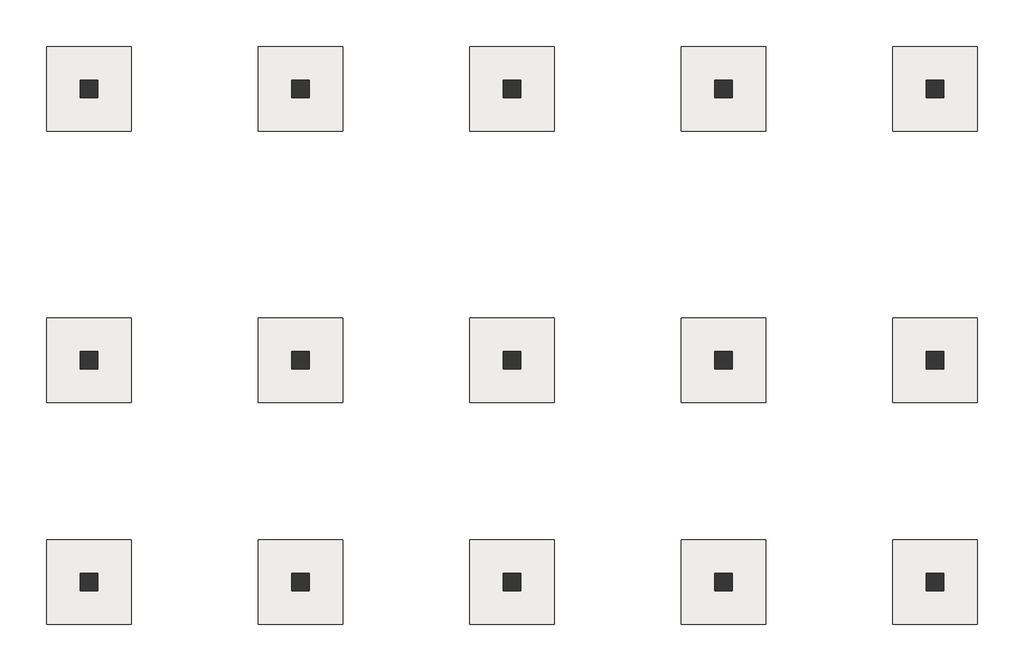
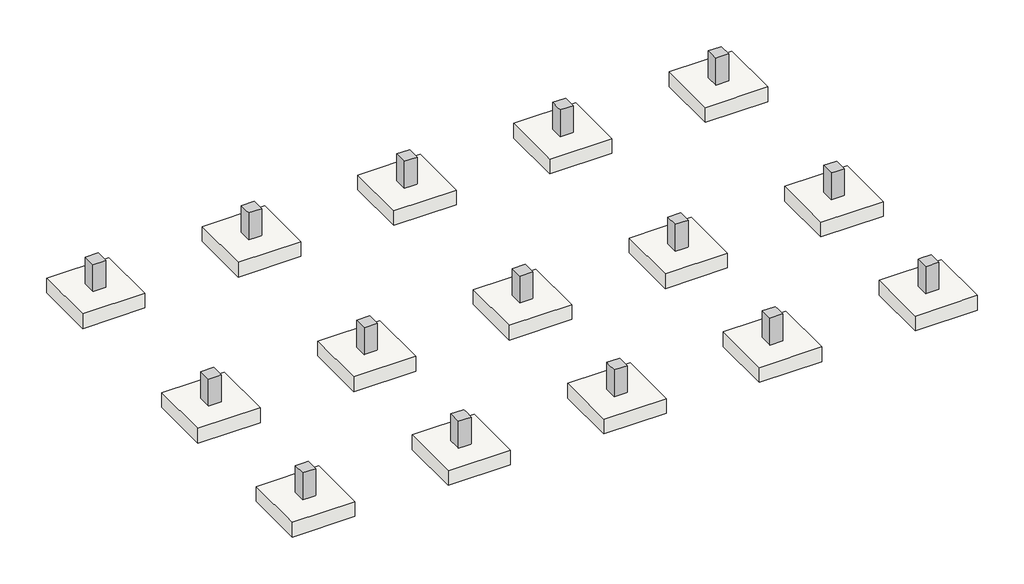
# One storey: 15 columns, 15 slabs.
"""IFC4 building model written with IfcOpenShell, lengths in millimetres."""

import ifcopenshell
import ifcopenshell.guid

model = None  # the IFC model being written
_history = None  # IfcOwnerHistory: only IFC2X3 demands one
_inside = {}  # id of a spatial element -> (the spatial element, [elements in it])
_under = {}  # id of a project, library or spatial element -> (it, [spatial elements below it])
_declared = {}  # id of a project -> (the project, [libraries it declares])
_typed = {}  # id of a type object -> (the type object, [elements of that type])
_made_of = {}  # id of a material, layer set ... -> (it, [elements and type objects made of it])


def new_model(schema):
    """Start an empty IFC model of exactly this schema.

    Asked for "IFC4X3", IfcOpenShell would pick the latest addendum, in which some entities
    have other attributes; the version numbers below select the first issue.
    IFC2X3 requires an IfcOwnerHistory on every rooted entity: one is made here for all.
    """
    global model, _history
    if schema == "IFC4X3":
        model = ifcopenshell.file(schema_version=(4, 3, 0, 0))
    else:
        model = ifcopenshell.file(schema=schema)
    _inside.clear()
    _under.clear()
    _declared.clear()
    _typed.clear()
    _made_of.clear()
    _history = None
    if model.schema == "IFC2X3":
        org = make("IfcOrganization", Name="unknown")
        user = make(
            "IfcPersonAndOrganization",
            ThePerson=make("IfcPerson", FamilyName="unknown"),
            TheOrganization=org,
        )
        app = make(
            "IfcApplication",
            ApplicationDeveloper=org,
            Version="unknown",
            ApplicationFullName="unknown",
            ApplicationIdentifier="unknown",
        )
        _history = make(
            "IfcOwnerHistory",
            OwningUser=user,
            OwningApplication=app,
            ChangeAction="ADDED",
            CreationDate=0,
        )
    return model


def make(cls, **values):
    """One entity of the class cls with the attributes given. An attribute that is None is left unset."""
    return model.create_entity(
        cls, **{name: value for name, value in values.items() if value is not None}
    )


def rooted(cls, **values):
    """An entity with a GlobalId (a new one), such as an element, a storey or a relation."""
    return make(cls, GlobalId=ifcopenshell.guid.new(), OwnerHistory=_history, **values)


def si_unit(unit_type, name, prefix=None):
    """IfcSIUnit, for example si_unit("LENGTHUNIT", "METRE", prefix="MILLI")."""
    return make("IfcSIUnit", UnitType=unit_type, Prefix=prefix, Name=name)


def assignment(units):
    """IfcUnitAssignment: the units of a project."""
    return None if units is None else make("IfcUnitAssignment", Units=units)


def point(xyz):
    """IfcCartesianPoint."""
    return None if xyz is None else make("IfcCartesianPoint", Coordinates=xyz)


def direction(xyz):
    """IfcDirection."""
    return None if xyz is None else make("IfcDirection", DirectionRatios=xyz)


def frame(location, z_axis=None, x_axis=None):
    """IfcAxis2Placement3D, a coordinate frame: its origin and axes. An axis left out is left unset."""
    return make(
        "IfcAxis2Placement3D",
        Location=point(location),
        Axis=direction(z_axis),
        RefDirection=direction(x_axis),
    )


def origin():
    """The frame at (0, 0, 0) with its axes left unset."""
    return frame((0.0, 0.0, 0.0))


def place(relative_to, where):
    """IfcLocalPlacement: puts the frame where relative to a parent placement (None: the world)."""
    return make(
        "IfcLocalPlacement", PlacementRelTo=relative_to, RelativePlacement=where
    )


def context(
    kind, dimensions, precision=None, world=None, true_north=None, identifier=None
):
    """IfcGeometricRepresentationContext, for example the 3D "Model" context."""
    return make(
        "IfcGeometricRepresentationContext",
        ContextIdentifier=identifier,
        ContextType=kind,
        CoordinateSpaceDimension=dimensions,
        Precision=precision,
        WorldCoordinateSystem=world,
        TrueNorth=true_north,
    )


def project(units=None, contexts=None):
    """IfcProject with its units and contexts."""
    return rooted(
        "IfcProject",
        Name="project",
        RepresentationContexts=contexts,
        UnitsInContext=assignment(units),
    )


def spatial(cls, under=None, at=None, **own):
    """A site, building, storey or space (cls), placed at a placement, below another one or the project."""
    s = rooted(cls, ObjectPlacement=at, **own)
    if under is not None:
        _under.setdefault(under.id(), (under, []))[1].append(s)
    return s


def polyline(points):
    """IfcPolyline through the points."""
    return make("IfcPolyline", Points=[point(p) for p in points])


def outline(outer, holes=None, kind="AREA"):
    """IfcArbitraryClosedProfileDef: a profile drawn as a closed curve; with holes, ...WithVoids."""
    if holes is None:
        return make("IfcArbitraryClosedProfileDef", ProfileType=kind, OuterCurve=outer)
    return make(
        "IfcArbitraryProfileDefWithVoids",
        ProfileType=kind,
        OuterCurve=outer,
        InnerCurves=holes,
    )


def extrude(swept, where, along, depth):
    """IfcExtrudedAreaSolid: the profile swept, set in the frame where, extruded along a direction by depth."""
    return make(
        "IfcExtrudedAreaSolid",
        SweptArea=swept,
        Position=where,
        ExtrudedDirection=direction(along),
        Depth=depth,
    )


def faces_of(points, faces, orient=None, outer=None):
    """IfcFace entities. A face is a list of loops; a loop is a list of indices into points, from 0.

    orient and outer hold one flag for each loop. By default every Orientation is true, the
    first loop of a face is its IfcFaceOuterBound and the others are IfcFaceBound.
    """
    made = []
    for i, loops in enumerate(faces):
        bounds = []
        for j, loop in enumerate(loops):
            is_outer = j == 0 if outer is None else outer[i][j]
            bounds.append(
                make(
                    "IfcFaceOuterBound" if is_outer else "IfcFaceBound",
                    Bound=make("IfcPolyLoop", Polygon=[points[k] for k in loop]),
                    Orientation=True if orient is None else orient[i][j],
                )
            )
        made.append(make("IfcFace", Bounds=bounds))
    return made


def faceted_brep(points, faces, orient=None, outer=None, voids=None):
    """IfcFacetedBrep: a solid bounded by flat faces; with voids (closed shells), ...WithVoids."""
    shared = [point(p) for p in points]
    hull = make("IfcClosedShell", CfsFaces=faces_of(shared, faces, orient, outer))
    if voids is None:
        return make("IfcFacetedBrep", Outer=hull)
    return make(
        "IfcFacetedBrepWithVoids",
        Outer=hull,
        Voids=[
            make(cls, CfsFaces=faces_of(shared, fs, o, b)) for cls, fs, o, b in voids
        ],
    )


def shape(context_of_items, identifier, shape_type, items):
    """IfcShapeRepresentation: the items that make up one representation, for example the "Body"."""
    return make(
        "IfcShapeRepresentation",
        ContextOfItems=context_of_items,
        RepresentationIdentifier=identifier,
        RepresentationType=shape_type,
        Items=items,
    )


def source(mapping_origin, context_of_items, identifier, shape_type, items):
    """IfcRepresentationMap: a shape defined once, which mapped items show again and again."""
    return make(
        "IfcRepresentationMap",
        MappingOrigin=mapping_origin,
        MappedRepresentation=shape(context_of_items, identifier, shape_type, items),
    )


def transform(
    local_origin,
    x_axis=None,
    y_axis=None,
    z_axis=None,
    scale=None,
    scale2=None,
    scale3=None,
    uniform=True,
):
    """IfcCartesianTransformationOperator3D, or its non-uniform kind. x_axis, y_axis, z_axis: its Axis1, 2, 3."""
    if uniform:
        return make(
            "IfcCartesianTransformationOperator3D",
            Axis1=direction(x_axis),
            Axis2=direction(y_axis),
            LocalOrigin=point(local_origin),
            Scale=scale,
            Axis3=direction(z_axis),
        )
    return make(
        "IfcCartesianTransformationOperator3DnonUniform",
        Axis1=direction(x_axis),
        Axis2=direction(y_axis),
        LocalOrigin=point(local_origin),
        Scale=scale,
        Axis3=direction(z_axis),
        Scale2=scale2,
        Scale3=scale3,
    )


def mapped(mapping_source, mapping_target):
    """IfcMappedItem: shows the shape of a source again, moved by a transform."""
    return make(
        "IfcMappedItem", MappingSource=mapping_source, MappingTarget=mapping_target
    )


def made_of(thing, what):
    """Note that an element or type object is made of a material, layer set ...; save() writes the relation."""
    if what is not None:
        _made_of.setdefault(what.id(), (what, []))[1].append(thing)
    return thing


def element(
    cls,
    number,
    at=None,
    inside=None,
    cuts=None,
    type_object=None,
    material=None,
    context=None,
    identifier="Body",
    shape_type=None,
    held_by="IfcProductDefinitionShape",
    body=None,
    shapes=None,
    **own,
):
    """One element of the class cls, such as IfcWall. Its Tag is "e" and its number.

    at: its placement. inside: the storey or other place that contains it. cuts: it is an
    opening in that element (IfcRelVoidsElement). A single representation is given by context,
    identifier, shape_type and body (its items); several are given by shapes. held_by: the class
    of the entity that holds the representations. save() writes the other relations.
    """
    e = rooted(cls, Tag="e%d" % number, ObjectPlacement=at, **own)
    if body is not None:
        shapes = [shape(context, identifier, shape_type, body)]
    if shapes is not None:
        e.Representation = make(held_by, Representations=shapes)
    if inside is not None:
        _inside.setdefault(inside.id(), (inside, []))[1].append(e)
    if cuts is not None:
        rooted(
            "IfcRelVoidsElement", RelatingBuildingElement=cuts, RelatedOpeningElement=e
        )
    if type_object is not None:
        _typed.setdefault(type_object.id(), (type_object, []))[1].append(e)
    return made_of(e, material)


def aggregate(whole, parts):
    """IfcRelAggregates: a whole, such as a stair, and the parts it consists of."""
    return rooted("IfcRelAggregates", RelatingObject=whole, RelatedObjects=parts)


def save(model, path):
    """Write the relations noted so far, then the file.

    IfcRelAggregates (storeys below a building ...), IfcRelContainedInSpatialStructure (elements
    in a storey), IfcRelDefinesByType, IfcRelAssociatesMaterial and IfcRelDeclares: one each for
    every whole, place, type object, material and project.
    """
    for whole, parts in _under.values():
        aggregate(whole, parts)
    for where, things in _inside.values():
        rooted(
            "IfcRelContainedInSpatialStructure",
            RelatedElements=things,
            RelatingStructure=where,
        )
    for kind, things in _typed.values():
        rooted("IfcRelDefinesByType", RelatedObjects=things, RelatingType=kind)
    for what, things in _made_of.values():
        rooted("IfcRelAssociatesMaterial", RelatedObjects=things, RelatingMaterial=what)
    for by, libraries in _declared.values():
        rooted("IfcRelDeclares", RelatingContext=by, RelatedDefinitions=libraries)
    model.write(path)


def foundation_rectangular_non_pile_2400_x_2400_x_600mm_9fdc1d6b(model_context):
    return source(origin(), model_context, "Body", "SweptSolid", [
        extrude(outline(polyline([(1200.0, 1200.0), (1200.0, -1200.0), (-1200.0, -1200.0), (-1200.0, 1200.0), (1200.0, 1200.0)])), frame((0.0, 0.0, -600.0), z_axis=(0.0, 0.0, 1.0), x_axis=(1.0, 0.0, 0.0)), (0.0, 0.0, 1.0), 600.0),
    ])


model = new_model("IFC4")

# Units and contexts
model_context = context("Model", 3, world=origin())
ifc_project = project(units=[si_unit("LENGTHUNIT", "METRE", prefix="MILLI")], contexts=[model_context])

# Site, building, storey
site = spatial("IfcSite", under=ifc_project)
building = spatial("IfcBuilding", under=site)
storey = spatial("IfcBuildingStorey", under=building, Name="BOF GL-1800", Elevation=-2000.0)

# Columns
placement = place(None, origin())
element("IfcColumn", 1, ObjectType="RC_Column_Rectangular : 500 x 500mm", at=placement, inside=storey, context=model_context, shape_type="Brep", body=[
    faceted_brep([(-18445.7273237, 9685.9763125, -1400.0), (-18445.7273237, 9185.9763125, -1400.0), (-18945.7273237, 9185.9763125, -1400.0), (-18945.7273237, 9685.9763125, -1400.0), (-18945.7273237, 9685.9763125, -300.0), (-18445.7273237, 9685.9763125, -300.0), (-18445.7273237, 9685.9763125, -700.0), (-18945.7273237, 9185.9763125, -700.0), (-18945.7273237, 9185.9763125, -300.0), (-18445.7273237, 9185.9763125, -300.0), (-18595.7273237, 9185.9763125, -300.0), (-18445.7273237, 9335.9763125, -300.0)], [[[0, 1, 2, 3]], [[0, 3, 4, 5, 6]], [[3, 2, 7, 8, 4]], [[2, 1, 9, 10, 8, 7]], [[1, 0, 6, 5, 11, 9]], [[5, 4, 8, 10, 9, 11]]]),
])
element("IfcColumn", 2, ObjectType="RC_Column_Rectangular : 500 x 500mm", at=placement, inside=storey, context=model_context, shape_type="Brep", body=[
    faceted_brep([(-18445.7273237, 1985.9763125, -1400.0), (-18445.7273237, 1485.9763125, -1400.0), (-18945.7273237, 1485.9763125, -1400.0), (-18945.7273237, 1985.9763125, -1400.0), (-18945.7273237, 1985.9763125, -300.0), (-18445.7273237, 1985.9763125, -300.0), (-18945.7273237, 1485.9763125, -700.0), (-18945.7273237, 1485.9763125, -300.0), (-18445.7273237, 1485.9763125, -300.0), (-18595.7273237, 1485.9763125, -300.0)], [[[0, 1, 2, 3]], [[0, 3, 4, 5]], [[3, 2, 6, 7, 4]], [[2, 1, 8, 9, 7, 6]], [[1, 0, 5, 8]], [[5, 4, 7, 9, 8]]]),
])
element("IfcColumn", 3, ObjectType="RC_Column_Rectangular : 500 x 500mm", at=placement, inside=storey, context=model_context, shape_type="Brep", body=[
    faceted_brep([(-18445.7273237, -4314.0236875, -1400.0), (-18445.7273237, -4814.0236875, -1400.0), (-18945.7273237, -4814.0236875, -1400.0), (-18945.7273237, -4314.0236875, -1400.0), (-18945.7273237, -4314.0236875, -700.0), (-18945.7273237, -4314.0236875, -300.0), (-18595.7273237, -4314.0236875, -300.0), (-18445.7273237, -4314.0236875, -300.0), (-18945.7273237, -4814.0236875, -300.0), (-18445.7273237, -4814.0236875, -700.0), (-18445.7273237, -4814.0236875, -300.0), (-18445.7273237, -4464.0236875, -300.0)], [[[0, 1, 2, 3]], [[0, 3, 4, 5, 6, 7]], [[3, 2, 8, 5, 4]], [[2, 1, 9, 10, 8]], [[1, 0, 7, 11, 10, 9]], [[7, 6, 5, 8, 10, 11]]]),
])
element("IfcColumn", 4, ObjectType="RC_Column_Rectangular : 500 x 500mm", at=placement, inside=storey, context=model_context, shape_type="Brep", body=[
    faceted_brep([(-12445.7273237, 9685.9763125, -1400.0), (-12445.7273237, 9185.9763125, -1400.0), (-12945.7273237, 9185.9763125, -1400.0), (-12945.7273237, 9685.9763125, -1400.0), (-12945.7273237, 9685.9763125, -700.0), (-12945.7273237, 9685.9763125, -300.0), (-12445.7273237, 9685.9763125, -300.0), (-12945.7273237, 9185.9763125, -300.0), (-12945.7273237, 9335.9763125, -300.0), (-12445.7273237, 9185.9763125, -300.0)], [[[0, 1, 2, 3]], [[0, 3, 4, 5, 6]], [[3, 2, 7, 8, 5, 4]], [[2, 1, 9, 7]], [[1, 0, 6, 9]], [[6, 5, 8, 7, 9]]]),
])
element("IfcColumn", 5, ObjectType="RC_Column_Rectangular : 500 x 500mm", at=placement, inside=storey, context=model_context, shape_type="SweptSolid", body=[
    extrude(outline(polyline([(-12445.7273237, 1985.9763125), (-12445.7273237, 1485.9763125), (-12945.7273237, 1485.9763125), (-12945.7273237, 1985.9763125), (-12445.7273237, 1985.9763125)])), frame((0.0, 0.0, -1400.0), z_axis=(0.0, 0.0, 1.0), x_axis=(1.0, 0.0, 0.0)), (0.0, 0.0, 1.0), 1100.0),
])
element("IfcColumn", 6, ObjectType="RC_Column_Rectangular : 500 x 500mm", at=placement, inside=storey, context=model_context, shape_type="Brep", body=[
    faceted_brep([(-12445.7273237, -4314.0236875, -1400.0), (-12445.7273237, -4814.0236875, -1400.0), (-12945.7273237, -4814.0236875, -1400.0), (-12945.7273237, -4314.0236875, -1400.0), (-12945.7273237, -4314.0236875, -300.0), (-12445.7273237, -4314.0236875, -300.0), (-12945.7273237, -4814.0236875, -700.0), (-12945.7273237, -4814.0236875, -300.0), (-12945.7273237, -4464.0236875, -300.0), (-12445.7273237, -4814.0236875, -700.0), (-12445.7273237, -4814.0236875, -300.0), (-12445.7273237, -4464.0236875, -300.0)], [[[0, 1, 2, 3]], [[0, 3, 4, 5]], [[3, 2, 6, 7, 8, 4]], [[2, 1, 9, 10, 7, 6]], [[1, 0, 5, 11, 10, 9]], [[5, 4, 8, 7, 10, 11]]]),
])
element("IfcColumn", 7, ObjectType="RC_Column_Rectangular : 500 x 500mm", at=placement, inside=storey, context=model_context, shape_type="Brep", body=[
    faceted_brep([(-6445.7273237, 9685.9763125, -1400.0), (-6445.7273237, 9185.9763125, -1400.0), (-6945.7273237, 9185.9763125, -1400.0), (-6945.7273237, 9685.9763125, -1400.0), (-6945.7273237, 9685.9763125, -700.0), (-6945.7273237, 9685.9763125, -300.0), (-6445.7273237, 9685.9763125, -300.0), (-6945.7273237, 9185.9763125, -300.0), (-6945.7273237, 9335.9763125, -300.0), (-6445.7273237, 9185.9763125, -300.0)], [[[0, 1, 2, 3]], [[0, 3, 4, 5, 6]], [[3, 2, 7, 8, 5, 4]], [[2, 1, 9, 7]], [[1, 0, 6, 9]], [[6, 5, 8, 7, 9]]]),
])
element("IfcColumn", 8, ObjectType="RC_Column_Rectangular : 500 x 500mm", at=placement, inside=storey, context=model_context, shape_type="SweptSolid", body=[
    extrude(outline(polyline([(-6445.7273237, 1985.9763125), (-6445.7273237, 1485.9763125), (-6945.7273237, 1485.9763125), (-6945.7273237, 1985.9763125), (-6445.7273237, 1985.9763125)])), frame((0.0, 0.0, -1400.0), z_axis=(0.0, 0.0, 1.0), x_axis=(1.0, 0.0, 0.0)), (0.0, 0.0, 1.0), 1100.0),
])
element("IfcColumn", 9, ObjectType="RC_Column_Rectangular : 500 x 500mm", at=placement, inside=storey, context=model_context, shape_type="Brep", body=[
    faceted_brep([(-6445.7273237, -4314.0236875, -1400.0), (-6445.7273237, -4814.0236875, -1400.0), (-6945.7273237, -4814.0236875, -1400.0), (-6945.7273237, -4314.0236875, -1400.0), (-6945.7273237, -4314.0236875, -300.0), (-6445.7273237, -4314.0236875, -300.0), (-6945.7273237, -4814.0236875, -700.0), (-6945.7273237, -4814.0236875, -300.0), (-6945.7273237, -4464.0236875, -300.0), (-6445.7273237, -4814.0236875, -700.0), (-6445.7273237, -4814.0236875, -300.0), (-6445.7273237, -4464.0236875, -300.0)], [[[0, 1, 2, 3]], [[0, 3, 4, 5]], [[3, 2, 6, 7, 8, 4]], [[2, 1, 9, 10, 7, 6]], [[1, 0, 5, 11, 10, 9]], [[5, 4, 8, 7, 10, 11]]]),
])
element("IfcColumn", 10, ObjectType="RC_Column_Rectangular : 500 x 500mm", at=placement, inside=storey, context=model_context, shape_type="Brep", body=[
    faceted_brep([(-445.7273237, 9685.9763125, -1400.0), (-445.7273237, 9185.9763125, -1400.0), (-945.7273237, 9185.9763125, -1400.0), (-945.7273237, 9685.9763125, -1400.0), (-945.7273237, 9685.9763125, -700.0), (-945.7273237, 9685.9763125, -300.0), (-445.7273237, 9685.9763125, -300.0), (-945.7273237, 9185.9763125, -300.0), (-945.7273237, 9335.9763125, -300.0), (-445.7273237, 9185.9763125, -300.0)], [[[0, 1, 2, 3]], [[0, 3, 4, 5, 6]], [[3, 2, 7, 8, 5, 4]], [[2, 1, 9, 7]], [[1, 0, 6, 9]], [[6, 5, 8, 7, 9]]]),
])
element("IfcColumn", 11, ObjectType="RC_Column_Rectangular : 500 x 500mm", at=placement, inside=storey, context=model_context, shape_type="SweptSolid", body=[
    extrude(outline(polyline([(-445.7273237, 1985.9763125), (-445.7273237, 1485.9763125), (-945.7273237, 1485.9763125), (-945.7273237, 1985.9763125), (-445.7273237, 1985.9763125)])), frame((0.0, 0.0, -1400.0), z_axis=(0.0, 0.0, 1.0), x_axis=(1.0, 0.0, 0.0)), (0.0, 0.0, 1.0), 1100.0),
])
element("IfcColumn", 12, ObjectType="RC_Column_Rectangular : 500 x 500mm", at=placement, inside=storey, context=model_context, shape_type="Brep", body=[
    faceted_brep([(-445.7273237, -4314.0236875, -1400.0), (-445.7273237, -4814.0236875, -1400.0), (-945.7273237, -4814.0236875, -1400.0), (-945.7273237, -4314.0236875, -1400.0), (-945.7273237, -4314.0236875, -300.0), (-445.7273237, -4314.0236875, -300.0), (-945.7273237, -4814.0236875, -700.0), (-945.7273237, -4814.0236875, -300.0), (-945.7273237, -4464.0236875, -300.0), (-445.7273237, -4814.0236875, -700.0), (-445.7273237, -4814.0236875, -300.0), (-445.7273237, -4464.0236875, -300.0)], [[[0, 1, 2, 3]], [[0, 3, 4, 5]], [[3, 2, 6, 7, 8, 4]], [[2, 1, 9, 10, 7, 6]], [[1, 0, 5, 11, 10, 9]], [[5, 4, 8, 7, 10, 11]]]),
])
element("IfcColumn", 13, ObjectType="RC_Column_Rectangular : 500 x 500mm", at=placement, inside=storey, context=model_context, shape_type="Brep", body=[
    faceted_brep([(5554.2726763, 9685.9763125, -1400.0), (5554.2726763, 9185.9763125, -1400.0), (5054.2726763, 9185.9763125, -1400.0), (5054.2726763, 9685.9763125, -1400.0), (5054.2726763, 9685.9763125, -700.0), (5054.2726763, 9685.9763125, -300.0), (5554.2726763, 9685.9763125, -300.0), (5054.2726763, 9185.9763125, -300.0), (5054.2726763, 9335.9763125, -300.0), (5554.2726763, 9185.9763125, -700.0), (5554.2726763, 9185.9763125, -300.0), (5204.2726763, 9185.9763125, -300.0)], [[[0, 1, 2, 3]], [[0, 3, 4, 5, 6]], [[3, 2, 7, 8, 5, 4]], [[2, 1, 9, 10, 11, 7]], [[1, 0, 6, 10, 9]], [[6, 5, 8, 7, 11, 10]]]),
])
element("IfcColumn", 14, ObjectType="RC_Column_Rectangular : 500 x 500mm", at=placement, inside=storey, context=model_context, shape_type="Brep", body=[
    faceted_brep([(5554.2726763, 1985.9763125, -1400.0), (5554.2726763, 1485.9763125, -1400.0), (5054.2726763, 1485.9763125, -1400.0), (5054.2726763, 1985.9763125, -1400.0), (5054.2726763, 1985.9763125, -300.0), (5554.2726763, 1985.9763125, -300.0), (5054.2726763, 1485.9763125, -300.0), (5554.2726763, 1485.9763125, -700.0), (5554.2726763, 1485.9763125, -300.0), (5204.2726763, 1485.9763125, -300.0)], [[[0, 1, 2, 3]], [[0, 3, 4, 5]], [[3, 2, 6, 4]], [[2, 1, 7, 8, 9, 6]], [[1, 0, 5, 8, 7]], [[5, 4, 6, 9, 8]]]),
])
element("IfcColumn", 15, ObjectType="RC_Column_Rectangular : 500 x 500mm", at=placement, inside=storey, context=model_context, shape_type="Brep", body=[
    faceted_brep([(5554.2726763, -4314.0236875, -1400.0), (5554.2726763, -4814.0236875, -1400.0), (5054.2726763, -4814.0236875, -1400.0), (5054.2726763, -4314.0236875, -1400.0), (5054.2726763, -4314.0236875, -300.0), (5204.2726763, -4314.0236875, -300.0), (5554.2726763, -4314.0236875, -300.0), (5554.2726763, -4314.0236875, -700.0), (5054.2726763, -4814.0236875, -700.0), (5054.2726763, -4814.0236875, -300.0), (5054.2726763, -4464.0236875, -300.0), (5554.2726763, -4814.0236875, -300.0)], [[[0, 1, 2, 3]], [[0, 3, 4, 5, 6, 7]], [[3, 2, 8, 9, 10, 4]], [[2, 1, 11, 9, 8]], [[1, 0, 7, 6, 11]], [[6, 5, 4, 10, 9, 11]]]),
])

# Slabs
foundation_rectangular_non_pile_2400_x_2400_x_600mm_shape = foundation_rectangular_non_pile_2400_x_2400_x_600mm_9fdc1d6b(model_context)
element("IfcSlab", 16, ObjectType="Foundation Rectangular(Non-Pile) : 2400 x 2400 x 600mm", at=placement, inside=storey, context=model_context, shape_type="MappedRepresentation", body=[
    mapped(foundation_rectangular_non_pile_2400_x_2400_x_600mm_shape, transform((-18695.7273237, 9435.9763125, -1400.0), x_axis=(1.0, 0.0, 0.0), y_axis=(0.0, 1.0, 0.0), z_axis=(0.0, 0.0, 1.0))),
])
element("IfcSlab", 17, ObjectType="Foundation Rectangular(Non-Pile) : 2400 x 2400 x 600mm", at=placement, inside=storey, context=model_context, shape_type="MappedRepresentation", body=[
    mapped(foundation_rectangular_non_pile_2400_x_2400_x_600mm_shape, transform((-18695.7273237, 1735.9763125, -1400.0), x_axis=(1.0, 0.0, 0.0), y_axis=(0.0, 1.0, 0.0), z_axis=(0.0, 0.0, 1.0))),
])
element("IfcSlab", 18, ObjectType="Foundation Rectangular(Non-Pile) : 2400 x 2400 x 600mm", at=placement, inside=storey, context=model_context, shape_type="MappedRepresentation", body=[
    mapped(foundation_rectangular_non_pile_2400_x_2400_x_600mm_shape, transform((-18695.7273237, -4564.0236875, -1400.0), x_axis=(1.0, 0.0, 0.0), y_axis=(0.0, 1.0, 0.0), z_axis=(0.0, 0.0, 1.0))),
])
element("IfcSlab", 19, ObjectType="Foundation Rectangular(Non-Pile) : 2400 x 2400 x 600mm", at=placement, inside=storey, context=model_context, shape_type="MappedRepresentation", body=[
    mapped(foundation_rectangular_non_pile_2400_x_2400_x_600mm_shape, transform((-12695.7273237, 9435.9763125, -1400.0), x_axis=(1.0, 0.0, 0.0), y_axis=(0.0, 1.0, 0.0), z_axis=(0.0, 0.0, 1.0))),
])
element("IfcSlab", 20, ObjectType="Foundation Rectangular(Non-Pile) : 2400 x 2400 x 600mm", at=placement, inside=storey, context=model_context, shape_type="MappedRepresentation", body=[
    mapped(foundation_rectangular_non_pile_2400_x_2400_x_600mm_shape, transform((-12695.7273237, 1735.9763125, -1400.0), x_axis=(1.0, 0.0, 0.0), y_axis=(0.0, 1.0, 0.0), z_axis=(0.0, 0.0, 1.0))),
])
element("IfcSlab", 21, ObjectType="Foundation Rectangular(Non-Pile) : 2400 x 2400 x 600mm", at=placement, inside=storey, context=model_context, shape_type="MappedRepresentation", body=[
    mapped(foundation_rectangular_non_pile_2400_x_2400_x_600mm_shape, transform((-12695.7273237, -4564.0236875, -1400.0), x_axis=(1.0, 0.0, 0.0), y_axis=(0.0, 1.0, 0.0), z_axis=(0.0, 0.0, 1.0))),
])
element("IfcSlab", 22, ObjectType="Foundation Rectangular(Non-Pile) : 2400 x 2400 x 600mm", at=placement, inside=storey, context=model_context, shape_type="MappedRepresentation", body=[
    mapped(foundation_rectangular_non_pile_2400_x_2400_x_600mm_shape, transform((-6695.7273237, 9435.9763125, -1400.0), x_axis=(1.0, 0.0, 0.0), y_axis=(0.0, 1.0, 0.0), z_axis=(0.0, 0.0, 1.0))),
])
element("IfcSlab", 23, ObjectType="Foundation Rectangular(Non-Pile) : 2400 x 2400 x 600mm", at=placement, inside=storey, context=model_context, shape_type="MappedRepresentation", body=[
    mapped(foundation_rectangular_non_pile_2400_x_2400_x_600mm_shape, transform((-6695.7273237, 1735.9763125, -1400.0), x_axis=(1.0, 0.0, 0.0), y_axis=(0.0, 1.0, 0.0), z_axis=(0.0, 0.0, 1.0))),
])
element("IfcSlab", 24, ObjectType="Foundation Rectangular(Non-Pile) : 2400 x 2400 x 600mm", at=placement, inside=storey, context=model_context, shape_type="MappedRepresentation", body=[
    mapped(foundation_rectangular_non_pile_2400_x_2400_x_600mm_shape, transform((-6695.7273237, -4564.0236875, -1400.0), x_axis=(1.0, 0.0, 0.0), y_axis=(0.0, 1.0, 0.0), z_axis=(0.0, 0.0, 1.0))),
])
element("IfcSlab", 25, ObjectType="Foundation Rectangular(Non-Pile) : 2400 x 2400 x 600mm", at=placement, inside=storey, context=model_context, shape_type="MappedRepresentation", body=[
    mapped(foundation_rectangular_non_pile_2400_x_2400_x_600mm_shape, transform((-695.7273237, 9435.9763125, -1400.0), x_axis=(1.0, 0.0, 0.0), y_axis=(0.0, 1.0, 0.0), z_axis=(0.0, 0.0, 1.0))),
])
element("IfcSlab", 26, ObjectType="Foundation Rectangular(Non-Pile) : 2400 x 2400 x 600mm", at=placement, inside=storey, context=model_context, shape_type="MappedRepresentation", body=[
    mapped(foundation_rectangular_non_pile_2400_x_2400_x_600mm_shape, transform((-695.7273237, 1735.9763125, -1400.0), x_axis=(1.0, 0.0, 0.0), y_axis=(0.0, 1.0, 0.0), z_axis=(0.0, 0.0, 1.0))),
])
element("IfcSlab", 27, ObjectType="Foundation Rectangular(Non-Pile) : 2400 x 2400 x 600mm", at=placement, inside=storey, context=model_context, shape_type="MappedRepresentation", body=[
    mapped(foundation_rectangular_non_pile_2400_x_2400_x_600mm_shape, transform((-695.7273237, -4564.0236875, -1400.0), x_axis=(1.0, 0.0, 0.0), y_axis=(0.0, 1.0, 0.0), z_axis=(0.0, 0.0, 1.0))),
])
element("IfcSlab", 28, ObjectType="Foundation Rectangular(Non-Pile) : 2400 x 2400 x 600mm", at=placement, inside=storey, context=model_context, shape_type="MappedRepresentation", body=[
    mapped(foundation_rectangular_non_pile_2400_x_2400_x_600mm_shape, transform((5304.2726763, 9435.9763125, -1400.0), x_axis=(1.0, 0.0, 0.0), y_axis=(0.0, 1.0, 0.0), z_axis=(0.0, 0.0, 1.0))),
])
element("IfcSlab", 29, ObjectType="Foundation Rectangular(Non-Pile) : 2400 x 2400 x 600mm", at=placement, inside=storey, context=model_context, shape_type="MappedRepresentation", body=[
    mapped(foundation_rectangular_non_pile_2400_x_2400_x_600mm_shape, transform((5304.2726763, 1735.9763125, -1400.0), x_axis=(1.0, 0.0, 0.0), y_axis=(0.0, 1.0, 0.0), z_axis=(0.0, 0.0, 1.0))),
])
element("IfcSlab", 30, ObjectType="Foundation Rectangular(Non-Pile) : 2400 x 2400 x 600mm", at=placement, inside=storey, context=model_context, shape_type="MappedRepresentation", body=[
    mapped(foundation_rectangular_non_pile_2400_x_2400_x_600mm_shape, transform((5304.2726763, -4564.0236875, -1400.0), x_axis=(1.0, 0.0, 0.0), y_axis=(0.0, 1.0, 0.0), z_axis=(0.0, 0.0, 1.0))),
])

save(model, "model.ifc")

# Revit data of these elements
# Project information
#   Project Issue Date = "발행 날짜"
#   Project Status = "프로젝트 상태"
#   Client Name = "소유자"
#   Project Address = "주소를 여기에 입력"
#   Project Name = "프로젝트 이름"
#   Project Number = "0001"
#   AreaCalculationInternationalBuildNumber = "ZgA=BAAAAA==2023BgFlAAAAAQgAAAABAQAAAAYBZAAAAAHnBwAABAQAAAABUAQAAAcH0"
#   BuildingbookInternationalBuildNumber = "ZgA=BAAAAA==2023BgFlAAAAAQoAAAABAQAAAAYBZAAAAAHnBwAABAQAAAABWwIAAAcH0"
#   RoomBookInternationalBuildNumber = "ZgA=BAAAAA==2023BgFlAAAAAQQAAAABAQAAAAYBZAAAAAHnBwAABAQAAAABTwQAAAcH1"
# Grids (mm)
#   "X2": line (-12695.727, -8233.19) -> (-12695.727, 14438.726)
#   "X3": line (-6695.727, -8233.19) -> (-6695.727, 14438.726)
#   "X4": line (-695.727, -8233.19) -> (-695.727, 14438.726)
#   "X5": line (5304.273, -8233.19) -> (5304.273, 14438.726)
#   "Y2": line (9794.388, 1735.976) -> (-24604.07, 1735.976)
#   "Y1": line (9794.388, -4564.024) -> (-24604.07, -4564.024)
#   "Y3": line (9794.388, 9435.976) -> (-24604.07, 9435.976)
#   "X1": line (-18695.727, -8233.19) -> (-18695.727, 14438.726)
#   "Y61": line (2304.273, -8233.19) -> (2304.273, 3037.902)
#   "Y62": line (9794.388, 4135.976) -> (-10544.455, 4135.976)
#   "Y63": line (-9695.727, 3037.902) -> (-9695.727, 14438.726)
# Type "RC_Column_Rectangular : 500 x 500mm"
#   b = 500 mm
#   h = 500 mm
#   Structural Material [instance default] = 콘크리트, 현장타설 회색
# Type "Foundation Rectangular(Non-Pile) : 2400 x 2400 x 600mm"
#   Width = 2400 mm
#   Length = 2400 mm
#   Foundation Thickness = 600 mm
#   Structural Material [instance default] = 콘크리트 - 현장타설 콘크리트
#   Assembly Code = ""
# Elements 1, 2, 3, 4, 5, 6, 7, 8, 9, 10, 11, 12, 13, 14, 15 (IfcColumn, "RC_Column_Rectangular : 500 x 500mm")
#   Structural Material = 콘크리트, 현장타설 회색
#   Phase Created = 신축
#   Materials on its faces: "콘크리트, 현장타설 회색"
# Elements 16, 17, 18, 19, 20, 21, 22, 23, 24, 25, 26, 27, 28, 29, 30 (IfcSlab, "Foundation Rectangular(Non-Pile) : 2400 x 2400 x 600mm")
#   Structural Material = 콘크리트 - 현장타설 콘크리트
#   Phase Created = 신축
#   Materials on its faces: "콘크리트 - 현장타설 콘크리트"
# Materials
#   "콘크리트, 현장타설 회색": class "콘크리트", colour RGB 192 192 192, transparency 0, Description = "현장타설 콘크리트", Cost = 0
#   "콘크리트 - 현장타설 콘크리트": class "콘크리트", colour RGB 192 192 192, transparency 0, Cost = 0
